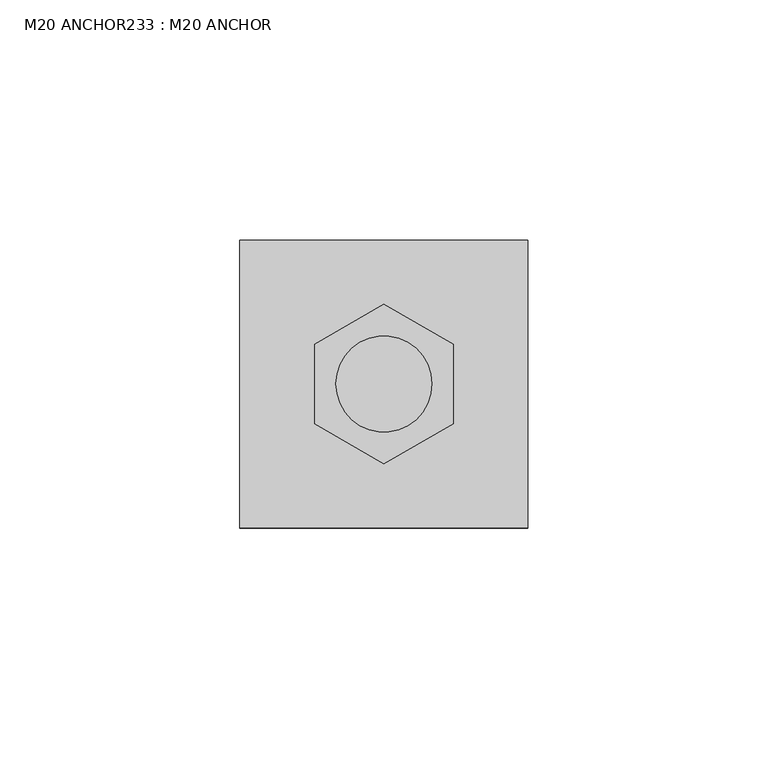
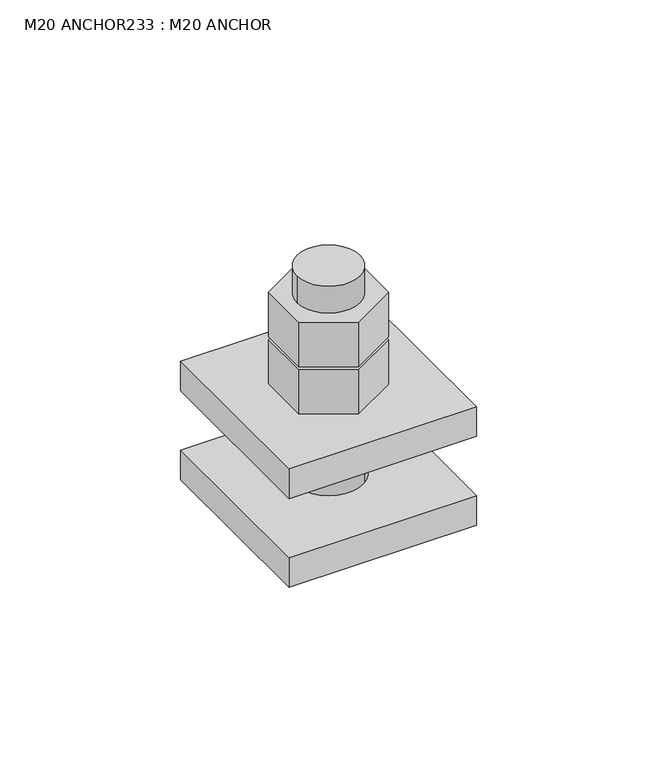
"""IFC4 building model written with IfcOpenShell, lengths in millimetres: fastener geometry, M20 ANCHOR233 : M20 ANCHOR."""

from ifc_helpers import new_model, si_unit, point, frame, frame_2d, origin, place, context, project, spatial, polyline, circle_curve, trimmed, segment, composite_curve, outline, extrude, source, transform, mapped, element, save


def m20_anchor233_m20_anchor_412aa66c(model_context):
    return source(origin(), model_context, "Body", "SweptSolid", [
        extrude(outline(polyline([(9008.0855968, 25545.0952779), (9022.4937158, 25553.4138093), (9036.9018348, 25545.0952779), (9036.9018348, 25528.4582151), (9022.4937158, 25520.1396837), (9008.0855968, 25528.4582151), (9008.0855968, 25545.0952779)]), holes=[composite_curve([segment(trimmed(circle_curve(frame_2d((9022.4937158, 25536.7767465)), 10.0), [point((9032.4937158, 25536.7767465))], [point((9012.4937158, 25536.7767465))], True, "CARTESIAN"), True, "CONTINUOUS"), segment(trimmed(circle_curve(frame_2d((9022.4937158, 25536.7767465)), 10.0), [point((9012.4937158, 25536.7767465))], [point((9032.4937158, 25536.7767465))], True, "CARTESIAN"), True, "CONTINUOUS")], self_intersect=False)]), frame((0.0, 0.0, 246.0), z_axis=(0.0, 0.0, 1.0), x_axis=(1.0, 0.0, 0.0)), (0.0, 0.0, 1.0), 15.0),
        extrude(outline(polyline([(9008.0855968, 25545.0952779), (9022.4937158, 25553.4138093), (9036.9018348, 25545.0952779), (9036.9018348, 25528.4582151), (9022.4937158, 25520.1396837), (9008.0855968, 25528.4582151), (9008.0855968, 25545.0952779)]), holes=[composite_curve([segment(trimmed(circle_curve(frame_2d((9022.4937158, 25536.7767465)), 10.0), [point((9032.4937158, 25536.7767465))], [point((9012.4937158, 25536.7767465))], True, "CARTESIAN"), True, "CONTINUOUS"), segment(trimmed(circle_curve(frame_2d((9022.4937158, 25536.7767465)), 10.0), [point((9012.4937158, 25536.7767465))], [point((9032.4937158, 25536.7767465))], True, "CARTESIAN"), True, "CONTINUOUS")], self_intersect=False)]), frame((0.0, 0.0, 230.0), z_axis=(0.0, 0.0, 1.0), x_axis=(1.0, 0.0, 0.0)), (0.0, 0.0, 1.0), 15.0),
        extrude(outline(composite_curve([segment(trimmed(circle_curve(frame_2d((9022.4937158, 25536.7767465)), 10.0), [point((9032.4937158, 25536.7767465))], [point((9012.4937158, 25536.7767465))], False, "CARTESIAN"), True, "CONTINUOUS"), segment(trimmed(circle_curve(frame_2d((9022.4937158, 25536.7767465)), 10.0), [point((9012.4937158, 25536.7767465))], [point((9032.4937158, 25536.7767465))], False, "CARTESIAN"), True, "CONTINUOUS")], self_intersect=False)), frame((0.0, 0.0, 190.0), z_axis=(0.0, 0.0, 1.0), x_axis=(1.0, 0.0, 0.0)), (0.0, 0.0, 1.0), 80.0),
        extrude(outline(polyline([(8992.4937158, 25566.7767465), (9052.4937158, 25566.7767465), (9052.4937158, 25506.7767465), (8992.4937158, 25506.7767465), (8992.4937158, 25566.7767465)]), holes=[composite_curve([segment(trimmed(circle_curve(frame_2d((9022.4937158, 25536.7767465)), 11.0), [point((9033.4937158, 25536.7767465))], [point((9011.4937158, 25536.7767465))], True, "CARTESIAN"), True, "CONTINUOUS"), segment(trimmed(circle_curve(frame_2d((9022.4937158, 25536.7767465)), 11.0), [point((9011.4937158, 25536.7767465))], [point((9033.4937158, 25536.7767465))], True, "CARTESIAN"), True, "CONTINUOUS")], self_intersect=False)]), frame((0.0, 0.0, 190.0), z_axis=(0.0, 0.0, 1.0), x_axis=(1.0, 0.0, 0.0)), (0.0, 0.0, 1.0), 10.0),
        extrude(outline(polyline([(8992.4937158, 25566.7767465), (9052.4937158, 25566.7767465), (9052.4937158, 25506.7767465), (8992.4937158, 25506.7767465), (8992.4937158, 25566.7767465)]), holes=[composite_curve([segment(trimmed(circle_curve(frame_2d((9022.4937158, 25536.7767465)), 11.0), [point((9033.4937158, 25536.7767465))], [point((9011.4937158, 25536.7767465))], True, "CARTESIAN"), True, "CONTINUOUS"), segment(trimmed(circle_curve(frame_2d((9022.4937158, 25536.7767465)), 11.0), [point((9011.4937158, 25536.7767465))], [point((9033.4937158, 25536.7767465))], True, "CARTESIAN"), True, "CONTINUOUS")], self_intersect=False)]), frame((0.0, 0.0, 220.0), z_axis=(0.0, 0.0, 1.0), x_axis=(1.0, 0.0, 0.0)), (0.0, 0.0, 1.0), 10.0),
    ])


if __name__ == "__main__":
    model = new_model("IFC4")
    model_context = context("Model", 3, world=origin())
    ifc_project = project(units=[si_unit("LENGTHUNIT", "METRE", prefix="MILLI")], contexts=[model_context])
    site = spatial("IfcSite", under=ifc_project)
    building = spatial("IfcBuilding", under=site)
    placement = place(None, origin())
    m20_anchor233_m20_anchor_shape = m20_anchor233_m20_anchor_412aa66c(model_context)
    element("IfcFastener", 1, ObjectType="M20 ANCHOR233 : M20 ANCHOR", at=placement, inside=building, context=model_context, shape_type="MappedRepresentation", body=[
        mapped(m20_anchor233_m20_anchor_shape, transform((0.0, 0.0, 0.0), x_axis=(1.0, 0.0, 0.0), y_axis=(0.0, 1.0, 0.0), z_axis=(0.0, 0.0, 1.0))),
    ])
    save(model, "model.ifc")
